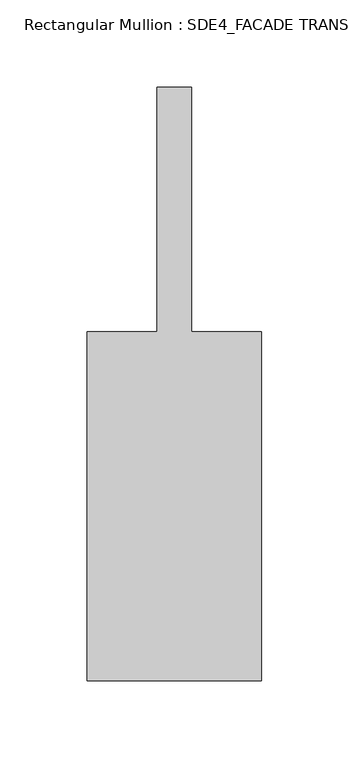
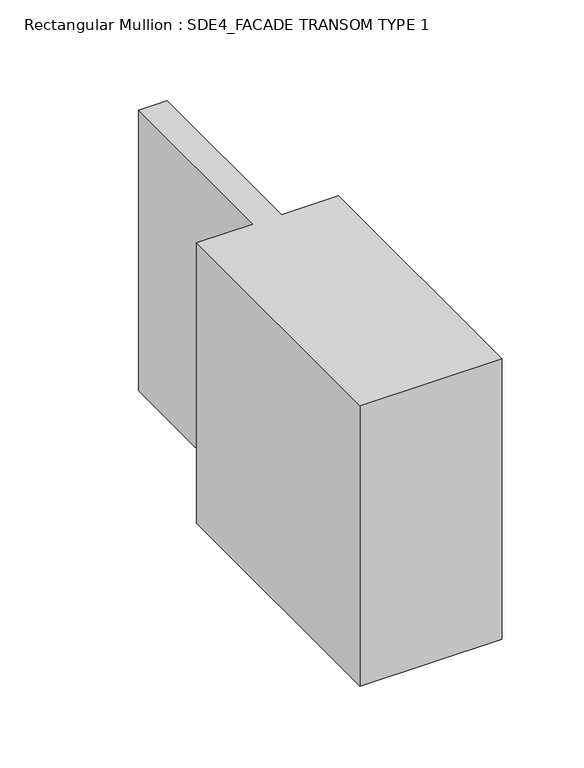
"""IFC4 building model written with IfcOpenShell, lengths in millimetres: member geometry, Rectangular Mullion : SDE4_FACADE TRANSOM TYPE 1."""

import ifcopenshell
import ifcopenshell.guid

model = None  # the IFC model being written
_history = None  # IfcOwnerHistory: only IFC2X3 demands one
_inside = {}  # id of a spatial element -> (the spatial element, [elements in it])
_under = {}  # id of a project, library or spatial element -> (it, [spatial elements below it])
_declared = {}  # id of a project -> (the project, [libraries it declares])
_typed = {}  # id of a type object -> (the type object, [elements of that type])
_made_of = {}  # id of a material, layer set ... -> (it, [elements and type objects made of it])


def new_model(schema):
    """Start an empty IFC model of exactly this schema.

    Asked for "IFC4X3", IfcOpenShell would pick the latest addendum, in which some entities
    have other attributes; the version numbers below select the first issue.
    IFC2X3 requires an IfcOwnerHistory on every rooted entity: one is made here for all.
    """
    global model, _history
    if schema == "IFC4X3":
        model = ifcopenshell.file(schema_version=(4, 3, 0, 0))
    else:
        model = ifcopenshell.file(schema=schema)
    _inside.clear()
    _under.clear()
    _declared.clear()
    _typed.clear()
    _made_of.clear()
    _history = None
    if model.schema == "IFC2X3":
        org = make("IfcOrganization", Name="unknown")
        user = make(
            "IfcPersonAndOrganization",
            ThePerson=make("IfcPerson", FamilyName="unknown"),
            TheOrganization=org,
        )
        app = make(
            "IfcApplication",
            ApplicationDeveloper=org,
            Version="unknown",
            ApplicationFullName="unknown",
            ApplicationIdentifier="unknown",
        )
        _history = make(
            "IfcOwnerHistory",
            OwningUser=user,
            OwningApplication=app,
            ChangeAction="ADDED",
            CreationDate=0,
        )
    return model


def make(cls, **values):
    """One entity of the class cls with the attributes given. An attribute that is None is left unset."""
    return model.create_entity(
        cls, **{name: value for name, value in values.items() if value is not None}
    )


def rooted(cls, **values):
    """An entity with a GlobalId (a new one), such as an element, a storey or a relation."""
    return make(cls, GlobalId=ifcopenshell.guid.new(), OwnerHistory=_history, **values)


def si_unit(unit_type, name, prefix=None):
    """IfcSIUnit, for example si_unit("LENGTHUNIT", "METRE", prefix="MILLI")."""
    return make("IfcSIUnit", UnitType=unit_type, Prefix=prefix, Name=name)


def assignment(units):
    """IfcUnitAssignment: the units of a project."""
    return None if units is None else make("IfcUnitAssignment", Units=units)


def point(xyz):
    """IfcCartesianPoint."""
    return None if xyz is None else make("IfcCartesianPoint", Coordinates=xyz)


def direction(xyz):
    """IfcDirection."""
    return None if xyz is None else make("IfcDirection", DirectionRatios=xyz)


def frame(location, z_axis=None, x_axis=None):
    """IfcAxis2Placement3D, a coordinate frame: its origin and axes. An axis left out is left unset."""
    return make(
        "IfcAxis2Placement3D",
        Location=point(location),
        Axis=direction(z_axis),
        RefDirection=direction(x_axis),
    )


def origin():
    """The frame at (0, 0, 0) with its axes left unset."""
    return frame((0.0, 0.0, 0.0))


def place(relative_to, where):
    """IfcLocalPlacement: puts the frame where relative to a parent placement (None: the world)."""
    return make(
        "IfcLocalPlacement", PlacementRelTo=relative_to, RelativePlacement=where
    )


def context(
    kind, dimensions, precision=None, world=None, true_north=None, identifier=None
):
    """IfcGeometricRepresentationContext, for example the 3D "Model" context."""
    return make(
        "IfcGeometricRepresentationContext",
        ContextIdentifier=identifier,
        ContextType=kind,
        CoordinateSpaceDimension=dimensions,
        Precision=precision,
        WorldCoordinateSystem=world,
        TrueNorth=true_north,
    )


def project(units=None, contexts=None):
    """IfcProject with its units and contexts."""
    return rooted(
        "IfcProject",
        Name="project",
        RepresentationContexts=contexts,
        UnitsInContext=assignment(units),
    )


def spatial(cls, under=None, at=None, **own):
    """A site, building, storey or space (cls), placed at a placement, below another one or the project."""
    s = rooted(cls, ObjectPlacement=at, **own)
    if under is not None:
        _under.setdefault(under.id(), (under, []))[1].append(s)
    return s


def polyline(points):
    """IfcPolyline through the points."""
    return make("IfcPolyline", Points=[point(p) for p in points])


def outline(outer, holes=None, kind="AREA"):
    """IfcArbitraryClosedProfileDef: a profile drawn as a closed curve; with holes, ...WithVoids."""
    if holes is None:
        return make("IfcArbitraryClosedProfileDef", ProfileType=kind, OuterCurve=outer)
    return make(
        "IfcArbitraryProfileDefWithVoids",
        ProfileType=kind,
        OuterCurve=outer,
        InnerCurves=holes,
    )


def extrude(swept, where, along, depth):
    """IfcExtrudedAreaSolid: the profile swept, set in the frame where, extruded along a direction by depth."""
    return make(
        "IfcExtrudedAreaSolid",
        SweptArea=swept,
        Position=where,
        ExtrudedDirection=direction(along),
        Depth=depth,
    )


def shape(context_of_items, identifier, shape_type, items):
    """IfcShapeRepresentation: the items that make up one representation, for example the "Body"."""
    return make(
        "IfcShapeRepresentation",
        ContextOfItems=context_of_items,
        RepresentationIdentifier=identifier,
        RepresentationType=shape_type,
        Items=items,
    )


def source(mapping_origin, context_of_items, identifier, shape_type, items):
    """IfcRepresentationMap: a shape defined once, which mapped items show again and again."""
    return make(
        "IfcRepresentationMap",
        MappingOrigin=mapping_origin,
        MappedRepresentation=shape(context_of_items, identifier, shape_type, items),
    )


def transform(
    local_origin,
    x_axis=None,
    y_axis=None,
    z_axis=None,
    scale=None,
    scale2=None,
    scale3=None,
    uniform=True,
):
    """IfcCartesianTransformationOperator3D, or its non-uniform kind. x_axis, y_axis, z_axis: its Axis1, 2, 3."""
    if uniform:
        return make(
            "IfcCartesianTransformationOperator3D",
            Axis1=direction(x_axis),
            Axis2=direction(y_axis),
            LocalOrigin=point(local_origin),
            Scale=scale,
            Axis3=direction(z_axis),
        )
    return make(
        "IfcCartesianTransformationOperator3DnonUniform",
        Axis1=direction(x_axis),
        Axis2=direction(y_axis),
        LocalOrigin=point(local_origin),
        Scale=scale,
        Axis3=direction(z_axis),
        Scale2=scale2,
        Scale3=scale3,
    )


def mapped(mapping_source, mapping_target):
    """IfcMappedItem: shows the shape of a source again, moved by a transform."""
    return make(
        "IfcMappedItem", MappingSource=mapping_source, MappingTarget=mapping_target
    )


def made_of(thing, what):
    """Note that an element or type object is made of a material, layer set ...; save() writes the relation."""
    if what is not None:
        _made_of.setdefault(what.id(), (what, []))[1].append(thing)
    return thing


def element(
    cls,
    number,
    at=None,
    inside=None,
    cuts=None,
    type_object=None,
    material=None,
    context=None,
    identifier="Body",
    shape_type=None,
    held_by="IfcProductDefinitionShape",
    body=None,
    shapes=None,
    **own,
):
    """One element of the class cls, such as IfcWall. Its Tag is "e" and its number.

    at: its placement. inside: the storey or other place that contains it. cuts: it is an
    opening in that element (IfcRelVoidsElement). A single representation is given by context,
    identifier, shape_type and body (its items); several are given by shapes. held_by: the class
    of the entity that holds the representations. save() writes the other relations.
    """
    e = rooted(cls, Tag="e%d" % number, ObjectPlacement=at, **own)
    if body is not None:
        shapes = [shape(context, identifier, shape_type, body)]
    if shapes is not None:
        e.Representation = make(held_by, Representations=shapes)
    if inside is not None:
        _inside.setdefault(inside.id(), (inside, []))[1].append(e)
    if cuts is not None:
        rooted(
            "IfcRelVoidsElement", RelatingBuildingElement=cuts, RelatedOpeningElement=e
        )
    if type_object is not None:
        _typed.setdefault(type_object.id(), (type_object, []))[1].append(e)
    return made_of(e, material)


def aggregate(whole, parts):
    """IfcRelAggregates: a whole, such as a stair, and the parts it consists of."""
    return rooted("IfcRelAggregates", RelatingObject=whole, RelatedObjects=parts)


def save(model, path):
    """Write the relations noted so far, then the file.

    IfcRelAggregates (storeys below a building ...), IfcRelContainedInSpatialStructure (elements
    in a storey), IfcRelDefinesByType, IfcRelAssociatesMaterial and IfcRelDeclares: one each for
    every whole, place, type object, material and project.
    """
    for whole, parts in _under.values():
        aggregate(whole, parts)
    for where, things in _inside.values():
        rooted(
            "IfcRelContainedInSpatialStructure",
            RelatedElements=things,
            RelatingStructure=where,
        )
    for kind, things in _typed.values():
        rooted("IfcRelDefinesByType", RelatedObjects=things, RelatingType=kind)
    for what, things in _made_of.values():
        rooted("IfcRelAssociatesMaterial", RelatedObjects=things, RelatingMaterial=what)
    for by, libraries in _declared.values():
        rooted("IfcRelDeclares", RelatingContext=by, RelatedDefinitions=libraries)
    model.write(path)


def rectangular_mullion_sde4_facade_transom_type_1_e9642041(model_context):
    return source(origin(), model_context, "Body", "SweptSolid", [
        extrude(outline(polyline([(50.0, -132.5), (-50.0, -132.5), (-50.0, 67.5), (-10.0, 67.5), (-10.0, 207.5), (10.0, 207.5), (10.0, 67.5), (50.0, 67.5), (50.0, -132.5)])), frame((0.0, 0.0, -208.9624711), z_axis=(0.0, 0.0, 1.0), x_axis=(1.0, 0.0, 0.0)), (0.0, 0.0, 1.0), 208.9624711),
    ])


if __name__ == "__main__":
    model = new_model("IFC4")
    model_context = context("Model", 3, world=origin())
    ifc_project = project(units=[si_unit("LENGTHUNIT", "METRE", prefix="MILLI")], contexts=[model_context])
    site = spatial("IfcSite", under=ifc_project)
    building = spatial("IfcBuilding", under=site)
    placement = place(None, origin())
    rectangular_mullion_sde4_facade_transom_type_1_shape = rectangular_mullion_sde4_facade_transom_type_1_e9642041(model_context)
    element("IfcMember", 1, ObjectType="Rectangular Mullion : SDE4_FACADE TRANSOM TYPE 1", at=placement, inside=building, context=model_context, shape_type="MappedRepresentation", body=[
        mapped(rectangular_mullion_sde4_facade_transom_type_1_shape, transform((0.0, 0.0, 0.0), x_axis=(1.0, 0.0, 0.0), y_axis=(0.0, 1.0, 0.0), z_axis=(0.0, 0.0, 1.0))),
    ])
    save(model, "model.ifc")

# Revit data of these elements
# Type "Rectangular Mullion : SDE4_FACADE TRANSOM TYPE 1"
#   built-in parameter 1007322 = 1.11549 (stored number, unit not read)
#   built-in parameter 1007321 = 0.164042 (stored number, unit not read)
#   built-in parameter 1007320 = 0.164042 (stored number, unit not read)
